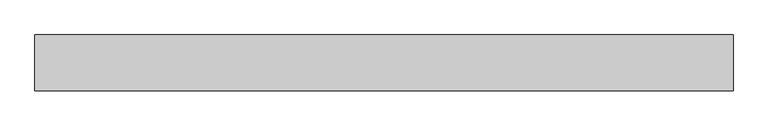
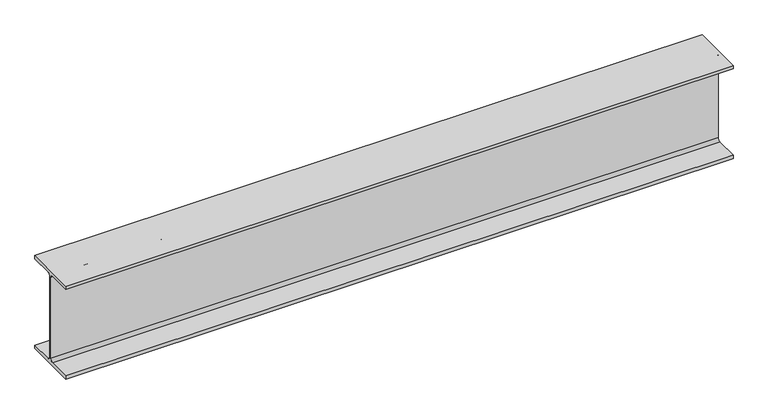
"""IFC4 building model written with IfcOpenShell, lengths in millimetres: beam geometry, Old_Steel Beam_H-KSD3502 : H_SB_ASB_H-194×150x6x9."""

import ifcopenshell
import ifcopenshell.guid

model = None  # the IFC model being written
_history = None  # IfcOwnerHistory: only IFC2X3 demands one
_inside = {}  # id of a spatial element -> (the spatial element, [elements in it])
_under = {}  # id of a project, library or spatial element -> (it, [spatial elements below it])
_declared = {}  # id of a project -> (the project, [libraries it declares])
_typed = {}  # id of a type object -> (the type object, [elements of that type])
_made_of = {}  # id of a material, layer set ... -> (it, [elements and type objects made of it])


def new_model(schema):
    """Start an empty IFC model of exactly this schema.

    Asked for "IFC4X3", IfcOpenShell would pick the latest addendum, in which some entities
    have other attributes; the version numbers below select the first issue.
    IFC2X3 requires an IfcOwnerHistory on every rooted entity: one is made here for all.
    """
    global model, _history
    if schema == "IFC4X3":
        model = ifcopenshell.file(schema_version=(4, 3, 0, 0))
    else:
        model = ifcopenshell.file(schema=schema)
    _inside.clear()
    _under.clear()
    _declared.clear()
    _typed.clear()
    _made_of.clear()
    _history = None
    if model.schema == "IFC2X3":
        org = make("IfcOrganization", Name="unknown")
        user = make(
            "IfcPersonAndOrganization",
            ThePerson=make("IfcPerson", FamilyName="unknown"),
            TheOrganization=org,
        )
        app = make(
            "IfcApplication",
            ApplicationDeveloper=org,
            Version="unknown",
            ApplicationFullName="unknown",
            ApplicationIdentifier="unknown",
        )
        _history = make(
            "IfcOwnerHistory",
            OwningUser=user,
            OwningApplication=app,
            ChangeAction="ADDED",
            CreationDate=0,
        )
    return model


def make(cls, **values):
    """One entity of the class cls with the attributes given. An attribute that is None is left unset."""
    return model.create_entity(
        cls, **{name: value for name, value in values.items() if value is not None}
    )


def rooted(cls, **values):
    """An entity with a GlobalId (a new one), such as an element, a storey or a relation."""
    return make(cls, GlobalId=ifcopenshell.guid.new(), OwnerHistory=_history, **values)


def si_unit(unit_type, name, prefix=None):
    """IfcSIUnit, for example si_unit("LENGTHUNIT", "METRE", prefix="MILLI")."""
    return make("IfcSIUnit", UnitType=unit_type, Prefix=prefix, Name=name)


def assignment(units):
    """IfcUnitAssignment: the units of a project."""
    return None if units is None else make("IfcUnitAssignment", Units=units)


def point(xyz):
    """IfcCartesianPoint."""
    return None if xyz is None else make("IfcCartesianPoint", Coordinates=xyz)


def direction(xyz):
    """IfcDirection."""
    return None if xyz is None else make("IfcDirection", DirectionRatios=xyz)


def frame(location, z_axis=None, x_axis=None):
    """IfcAxis2Placement3D, a coordinate frame: its origin and axes. An axis left out is left unset."""
    return make(
        "IfcAxis2Placement3D",
        Location=point(location),
        Axis=direction(z_axis),
        RefDirection=direction(x_axis),
    )


def frame_2d(location, x_axis=None):
    """IfcAxis2Placement2D, a coordinate frame in the plane: its origin and x axis."""
    return make(
        "IfcAxis2Placement2D", Location=point(location), RefDirection=direction(x_axis)
    )


def origin():
    """The frame at (0, 0, 0) with its axes left unset."""
    return frame((0.0, 0.0, 0.0))


def place(relative_to, where):
    """IfcLocalPlacement: puts the frame where relative to a parent placement (None: the world)."""
    return make(
        "IfcLocalPlacement", PlacementRelTo=relative_to, RelativePlacement=where
    )


def context(
    kind, dimensions, precision=None, world=None, true_north=None, identifier=None
):
    """IfcGeometricRepresentationContext, for example the 3D "Model" context."""
    return make(
        "IfcGeometricRepresentationContext",
        ContextIdentifier=identifier,
        ContextType=kind,
        CoordinateSpaceDimension=dimensions,
        Precision=precision,
        WorldCoordinateSystem=world,
        TrueNorth=true_north,
    )


def project(units=None, contexts=None):
    """IfcProject with its units and contexts."""
    return rooted(
        "IfcProject",
        Name="project",
        RepresentationContexts=contexts,
        UnitsInContext=assignment(units),
    )


def spatial(cls, under=None, at=None, **own):
    """A site, building, storey or space (cls), placed at a placement, below another one or the project."""
    s = rooted(cls, ObjectPlacement=at, **own)
    if under is not None:
        _under.setdefault(under.id(), (under, []))[1].append(s)
    return s


def polyline(points):
    """IfcPolyline through the points."""
    return make("IfcPolyline", Points=[point(p) for p in points])


def circle_curve(where, radius):
    """IfcCircle in the frame where."""
    return make("IfcCircle", Position=where, Radius=radius)


def trimmed(basis, trim1, trim2, sense, master):
    """IfcTrimmedCurve: the piece of a basis curve between two trims."""
    return make(
        "IfcTrimmedCurve",
        BasisCurve=basis,
        Trim1=trim1,
        Trim2=trim2,
        SenseAgreement=sense,
        MasterRepresentation=master,
    )


def segment(curve, same_sense, transition):
    """IfcCompositeCurveSegment."""
    return make(
        "IfcCompositeCurveSegment",
        Transition=transition,
        SameSense=same_sense,
        ParentCurve=curve,
    )


def composite_curve(segments, self_intersect=None):
    """IfcCompositeCurve: segments joined end to end."""
    return make("IfcCompositeCurve", Segments=segments, SelfIntersect=self_intersect)


def outline(outer, holes=None, kind="AREA"):
    """IfcArbitraryClosedProfileDef: a profile drawn as a closed curve; with holes, ...WithVoids."""
    if holes is None:
        return make("IfcArbitraryClosedProfileDef", ProfileType=kind, OuterCurve=outer)
    return make(
        "IfcArbitraryProfileDefWithVoids",
        ProfileType=kind,
        OuterCurve=outer,
        InnerCurves=holes,
    )


def extrude(swept, where, along, depth):
    """IfcExtrudedAreaSolid: the profile swept, set in the frame where, extruded along a direction by depth."""
    return make(
        "IfcExtrudedAreaSolid",
        SweptArea=swept,
        Position=where,
        ExtrudedDirection=direction(along),
        Depth=depth,
    )


def shape(context_of_items, identifier, shape_type, items):
    """IfcShapeRepresentation: the items that make up one representation, for example the "Body"."""
    return make(
        "IfcShapeRepresentation",
        ContextOfItems=context_of_items,
        RepresentationIdentifier=identifier,
        RepresentationType=shape_type,
        Items=items,
    )


def source(mapping_origin, context_of_items, identifier, shape_type, items):
    """IfcRepresentationMap: a shape defined once, which mapped items show again and again."""
    return make(
        "IfcRepresentationMap",
        MappingOrigin=mapping_origin,
        MappedRepresentation=shape(context_of_items, identifier, shape_type, items),
    )


def transform(
    local_origin,
    x_axis=None,
    y_axis=None,
    z_axis=None,
    scale=None,
    scale2=None,
    scale3=None,
    uniform=True,
):
    """IfcCartesianTransformationOperator3D, or its non-uniform kind. x_axis, y_axis, z_axis: its Axis1, 2, 3."""
    if uniform:
        return make(
            "IfcCartesianTransformationOperator3D",
            Axis1=direction(x_axis),
            Axis2=direction(y_axis),
            LocalOrigin=point(local_origin),
            Scale=scale,
            Axis3=direction(z_axis),
        )
    return make(
        "IfcCartesianTransformationOperator3DnonUniform",
        Axis1=direction(x_axis),
        Axis2=direction(y_axis),
        LocalOrigin=point(local_origin),
        Scale=scale,
        Axis3=direction(z_axis),
        Scale2=scale2,
        Scale3=scale3,
    )


def mapped(mapping_source, mapping_target):
    """IfcMappedItem: shows the shape of a source again, moved by a transform."""
    return make(
        "IfcMappedItem", MappingSource=mapping_source, MappingTarget=mapping_target
    )


def made_of(thing, what):
    """Note that an element or type object is made of a material, layer set ...; save() writes the relation."""
    if what is not None:
        _made_of.setdefault(what.id(), (what, []))[1].append(thing)
    return thing


def element(
    cls,
    number,
    at=None,
    inside=None,
    cuts=None,
    type_object=None,
    material=None,
    context=None,
    identifier="Body",
    shape_type=None,
    held_by="IfcProductDefinitionShape",
    body=None,
    shapes=None,
    **own,
):
    """One element of the class cls, such as IfcWall. Its Tag is "e" and its number.

    at: its placement. inside: the storey or other place that contains it. cuts: it is an
    opening in that element (IfcRelVoidsElement). A single representation is given by context,
    identifier, shape_type and body (its items); several are given by shapes. held_by: the class
    of the entity that holds the representations. save() writes the other relations.
    """
    e = rooted(cls, Tag="e%d" % number, ObjectPlacement=at, **own)
    if body is not None:
        shapes = [shape(context, identifier, shape_type, body)]
    if shapes is not None:
        e.Representation = make(held_by, Representations=shapes)
    if inside is not None:
        _inside.setdefault(inside.id(), (inside, []))[1].append(e)
    if cuts is not None:
        rooted(
            "IfcRelVoidsElement", RelatingBuildingElement=cuts, RelatedOpeningElement=e
        )
    if type_object is not None:
        _typed.setdefault(type_object.id(), (type_object, []))[1].append(e)
    return made_of(e, material)


def aggregate(whole, parts):
    """IfcRelAggregates: a whole, such as a stair, and the parts it consists of."""
    return rooted("IfcRelAggregates", RelatingObject=whole, RelatedObjects=parts)


def save(model, path):
    """Write the relations noted so far, then the file.

    IfcRelAggregates (storeys below a building ...), IfcRelContainedInSpatialStructure (elements
    in a storey), IfcRelDefinesByType, IfcRelAssociatesMaterial and IfcRelDeclares: one each for
    every whole, place, type object, material and project.
    """
    for whole, parts in _under.values():
        aggregate(whole, parts)
    for where, things in _inside.values():
        rooted(
            "IfcRelContainedInSpatialStructure",
            RelatedElements=things,
            RelatingStructure=where,
        )
    for kind, things in _typed.values():
        rooted("IfcRelDefinesByType", RelatedObjects=things, RelatingType=kind)
    for what, things in _made_of.values():
        rooted("IfcRelAssociatesMaterial", RelatedObjects=things, RelatingMaterial=what)
    for by, libraries in _declared.values():
        rooted("IfcRelDeclares", RelatingContext=by, RelatedDefinitions=libraries)
    model.write(path)


def beam_6061688a(model_context):
    return source(origin(), model_context, "Body", "SweptSolid", [
        extrude(outline(composite_curve([segment(polyline([(-82.5, -141.5), (-11.9, -141.5)]), True, "CONTINUOUS"), segment(trimmed(circle_curve(frame_2d((-11.9, -132.6)), 8.9), [point((-11.9, -141.5))], [point((-3.0, -132.6))], True, "CARTESIAN"), True, "CONTINUOUS"), segment(polyline([(-3.0, -132.6), (-3.0, 132.6)]), True, "CONTINUOUS"), segment(trimmed(circle_curve(frame_2d((-11.9, 132.6)), 8.9), [point((-3.0, 132.6))], [point((-11.9, 141.5))], True, "CARTESIAN"), True, "CONTINUOUS"), segment(polyline([(-11.9, 141.5), (-82.5, 141.5), (-82.5, 151.7), (82.5, 151.7), (82.5, 141.5), (11.9, 141.5)]), True, "CONTINUOUS"), segment(trimmed(circle_curve(frame_2d((11.9, 132.6)), 8.9), [point((11.9, 141.5))], [point((3.0, 132.6))], True, "CARTESIAN"), True, "CONTINUOUS"), segment(polyline([(3.0, 132.6), (3.0, -132.6)]), True, "CONTINUOUS"), segment(trimmed(circle_curve(frame_2d((11.9, -132.6)), 8.9), [point((3.0, -132.6))], [point((11.9, -141.5))], True, "CARTESIAN"), True, "CONTINUOUS"), segment(polyline([(11.9, -141.5), (82.5, -141.5), (82.5, -151.7), (-82.5, -151.7), (-82.5, -141.5)]), True, "CONTINUOUS")], self_intersect=False)), frame((-1047.9231301, 0.0, 0.0), z_axis=(1.0, 0.0, 0.0), x_axis=(0.0, 1.0, 0.0)), (0.0, 0.0, 1.0), 2060.1030758),
    ])


if __name__ == "__main__":
    model = new_model("IFC4")
    model_context = context("Model", 3, world=origin())
    ifc_project = project(units=[si_unit("LENGTHUNIT", "METRE", prefix="MILLI")], contexts=[model_context])
    site = spatial("IfcSite", under=ifc_project)
    building = spatial("IfcBuilding", under=site)
    placement = place(None, origin())
    beam_shape = beam_6061688a(model_context)
    element("IfcBeam", 1, ObjectType="Old_Steel Beam_H-KSD3502 : H_SB_ASB_H-194×150x6x9", at=placement, inside=building, context=model_context, shape_type="MappedRepresentation", body=[
        mapped(beam_shape, transform((0.0, 0.0, 0.0), x_axis=(1.0, 0.0, 0.0), y_axis=(0.0, 1.0, 0.0), z_axis=(0.0, 0.0, 1.0))),
    ])
    save(model, "model.ifc")

# Revit data of these elements
# Type "Old_Steel Beam_H-KSD3502 : H_SB_ASB_H-194×150x6x9"
#   Width = 15.0 cm
#   Web Thickness = 0.6 cm
#   Web Fillet = 1.3 cm
#   Warping Constant = 43316.0 cm⁶
#   Torsional Moment of Inertia = 8.622 cm⁴
#   Torsional Modulus = 1.0 cm³
#   Section Area = 39.01 cm²
#   Plastic Modulus weak axis = 104.0 cm³
#   Plastic Modulus strong axis = 309.0 cm³
#   Perimeter = 0.95 m²/m
#   Nominal Weight = 30.60 kgf/m
#   Moment of Inertia weak axis = 507.00 cm⁴
#   Moment of Inertia strong axis = 2690.00 cm⁴
#   Height = 19.4 cm
#   Flange Thickness = 0.9 cm
#   Elastic Modulus weak axis = 67.6 cm³
#   Elastic Modulus strong axis = 277.0 cm³
#   Centroid Vertical = 9.7 cm
#   Centroid Horizontal = 7.5 cm
#   Length [instance default] = 1.5240 m
#   Structural Material [instance default] = Steel, 45-345
#   Assembly Code = ""
# Element 1 (IfcBeam, "Old_Steel Beam_H-KSD3502 : H_SB_ASB_H-194×150x6x9")
#   Structural Material = none
# Materials
#   "Steel, 45-345": class "Metal", colour RGB 189 187 185, transparency 0, Description = "Steel 345 MPa", Cost = 0
